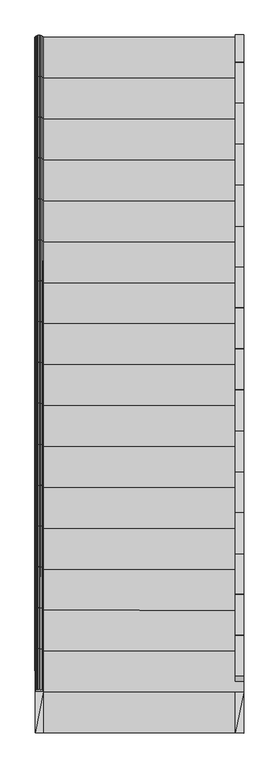
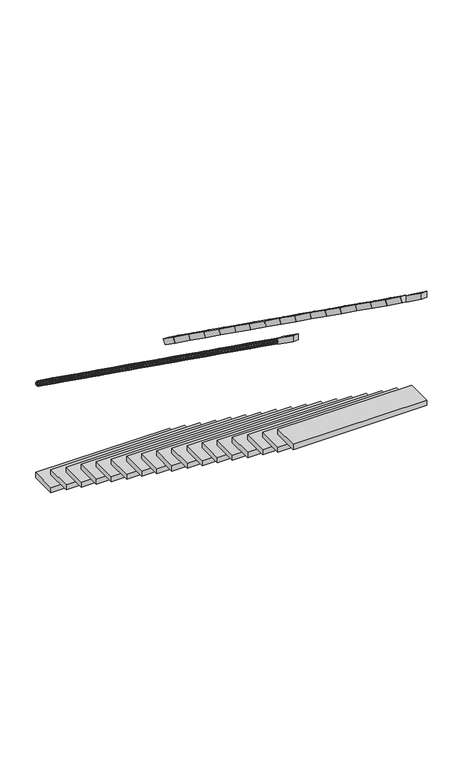
"""IFC4 building model written with IfcOpenShell, lengths in millimetres: stair geometry, 0_3d_modell."""

from ifc_helpers import new_model, si_unit, frame, origin, origin_with_axes, place, context, project, spatial, polyline, outline, extrude, faceted_brep, source, transform, mapped, element, save


def stair_c8e6e2fb(model_context):
    return source(origin(), model_context, "Body", "SolidModel", [
        extrude(outline(polyline([(1249.8201376, 2937.4233037), (1249.7841678, 2692.4712959), (0.2158186, 2693.7650028), (0.1798488, 2938.4708402), (1249.8201376, 2937.4233037)])), frame((0.0, 0.0, 875.0), z_axis=(0.0, 0.0, 1.0), x_axis=(1.0, 0.0, 0.0)), (0.0, 0.0, 1.0), 50.0),
        faceted_brep([(1.6558478, 1221.2875213, 3015.1503975), (0.4316459, 1225.4705658, 3021.0), (1.654618, 1229.65397, 3026.8496025), (5.2050513, 1233.4282332, 3032.1266051), (10.7354046, 1236.4239042, 3036.3144581), (17.7043284, 1238.3477458, 3039.0032253), (25.4296557, 1239.011439, 3039.9297113), (33.1551779, 1238.3500169, 3039.0032253), (40.1246669, 1236.4282241, 3036.3144581), (45.6559006, 1233.4341791, 3032.1266051), (49.2074433, 1229.6609599, 3026.8496025), (50.4316453, 1225.4779154, 3021.0), (49.2086731, 1221.2945111, 3015.1503975), (45.6582398, 1217.520248, 3009.8733949), (40.1278866, 1214.524577, 3005.6855419), (33.1589628, 1212.6007354, 3002.9967747), (25.4336355, 1211.9370421, 3002.0702887), (17.7081133, 1212.5984642, 3002.9967747), (10.7386243, 1214.520257, 3005.6855419), (5.2073906, 1217.514302, 3009.8733949), (1.6905885, 984.9431074, 3201.8496026), (0.4676164, 980.7597033, 3196.0), (1.6918183, 976.5766589, 3190.1503974), (5.2433611, 972.8034398, 3184.8733946), (10.7745948, 969.8093949, 3180.6855416), (17.7440838, 967.8876022, 3177.9967744), (25.469606, 967.2261802, 3177.0702883), (33.1949333, 967.8898734, 3177.9967744), (40.1638571, 969.8137149, 3180.6855416), (45.6942103, 972.8093858, 3184.8733946), (49.2446436, 976.5836488, 3190.1503974), (50.4676158, 980.7670529, 3196.0), (49.2434138, 984.9500972, 3201.8496026), (45.6918711, 988.7233163, 3207.1266054), (40.1606374, 991.7173612, 3211.3144584), (33.1911484, 993.6391539, 3214.0032256), (25.4656262, 994.300576, 3214.9297117), (17.7402989, 993.6368828, 3214.0032256), (10.7713751, 991.7130413, 3211.3144584), (5.2410218, 988.7173704, 3207.1266054)], [[[0, 1, 2, 3, 4, 5, 6, 7, 8, 9, 10, 11, 12, 13, 14, 15, 16, 17, 18, 19]], [[20, 21, 22, 23, 24, 25, 26, 27, 28, 29, 30, 31, 32, 33, 34, 35, 36, 37, 38, 39]], [[2, 1, 21, 20]], [[3, 2, 20, 39]], [[4, 3, 39, 38]], [[5, 4, 38, 37]], [[6, 5, 37, 36]], [[7, 6, 36, 35]], [[8, 7, 35, 34]], [[9, 8, 34, 33]], [[10, 9, 33, 32]], [[11, 10, 32, 31]], [[12, 11, 31, 30]], [[13, 12, 30, 29]], [[14, 13, 29, 28]], [[15, 14, 28, 27]], [[16, 15, 27, 26]], [[17, 16, 26, 25]], [[18, 17, 25, 24]], [[19, 18, 24, 23]], [[0, 19, 23, 22]], [[1, 0, 22, 21]]]),
        extrude(outline(polyline([(8.1923594, -49.3242866), (0.0, 0.0), (296.970001, 49.3242865), (305.1623617, 2e-07), (8.1923594, -49.3242866)])), frame((1249.7982535, 2788.3939483, 1932.2457474), z_axis=(-0.9999999892183942, 0.00014684417532646174, 0.0), x_axis=(-0.00013185516429988818, -0.8979257278461469, 0.44014698668306607)), (0.0, 0.0, 1.0), 50.0),
        extrude(outline(polyline([(8.1923603, -49.3242865), (0.0, 0.0), (296.9699661, 49.3242863), (305.1623277, 1e-07), (8.1923603, -49.3242865)])), frame((1249.6903463, 2053.5527853, 2457.2457396), z_axis=(-0.9999999892183942, 0.00014684417532705656, 0.0), x_axis=(-0.00013185516035039472, -0.897925700001221, 0.44014704348834854)), (0.0, 0.0, 1.0), 50.0),
        faceted_brep([(1.7637594, 487.1548921, 3540.1503972), (0.5395574, 491.3379361, 3546.0), (1.7625296, 495.5213399, 3551.8496028), (5.3129629, 499.2956026, 3557.1266058), (10.8433161, 502.2912733, 3561.314459), (17.8122399, 504.2151146, 3564.0032263), (25.5375672, 504.8788078, 3564.9297124), (33.2630894, 504.2173858, 3564.0032263), (40.2325784, 502.2955932, 3561.314459), (45.7638121, 499.3015486, 3557.1266058), (49.3153549, 495.5283297, 3551.8496028), (50.5395568, 491.3452857, 3546.0), (49.3165847, 487.161882, 3540.1503972), (45.7661514, 483.3876192, 3534.8733942), (40.2357981, 480.3919486, 3530.685541), (33.2668743, 478.4681072, 3527.9967737), (25.541547, 477.804414, 3527.0702876), (17.8160248, 478.465836, 3527.9967737), (10.8465358, 480.3876286, 3530.685541), (5.3153021, 483.3816732, 3534.8733942), (1.7985001, 250.810435, 3726.8496029), (0.5755279, 246.6270315, 3721.0), (1.7997299, 242.4439876, 3715.1503971), (5.3512726, 238.6707689, 3709.873394), (10.8825063, 235.6767243, 3705.6855407), (17.8519953, 233.7549319, 3702.9967733), (25.5775175, 233.0935099, 3702.0702872), (33.3028449, 233.757203, 3702.9967733), (40.2717686, 235.6810443, 3705.6855407), (45.8021219, 238.6767148, 3709.873394), (49.3525552, 242.4509775, 3715.1503971), (50.5755273, 246.634381, 3721.0), (49.3513254, 250.8174249, 3726.8496029), (45.7997826, 254.5906436, 3732.126606), (40.2685489, 257.5846882, 3736.3144593), (33.2990599, 259.5064806, 3739.0032267), (25.5735378, 260.1679026, 3739.9297128), (17.8482104, 259.5042095, 3739.0032267), (10.8792866, 257.5803682, 3736.3144593), (5.3489334, 254.5846977, 3732.126606)], [[[0, 1, 2, 3, 4, 5, 6, 7, 8, 9, 10, 11, 12, 13, 14, 15, 16, 17, 18, 19]], [[20, 21, 22, 23, 24, 25, 26, 27, 28, 29, 30, 31, 32, 33, 34, 35, 36, 37, 38, 39]], [[2, 1, 21, 20]], [[3, 2, 20, 39]], [[4, 3, 39, 38]], [[5, 4, 38, 37]], [[6, 5, 37, 36]], [[7, 6, 36, 35]], [[8, 7, 35, 34]], [[9, 8, 34, 33]], [[10, 9, 33, 32]], [[11, 10, 32, 31]], [[12, 11, 31, 30]], [[13, 12, 30, 29]], [[14, 13, 29, 28]], [[15, 14, 28, 27]], [[16, 15, 27, 26]], [[17, 16, 26, 25]], [[18, 17, 25, 24]], [[19, 18, 24, 23]], [[0, 19, 23, 22]], [[1, 0, 22, 21]]]),
        extrude(outline(polyline([(8.1923606, -49.3242864), (0.0, 0.0), (296.9699544, 49.3242862), (305.1623164, 1e-07), (8.1923606, -49.3242864)])), frame((1249.6543773, 1808.6057592, 2632.245737), z_axis=(-0.9999999892183942, 0.00014684417504094816, 0.0), x_axis=(-0.0001318551587321288, -0.8979256907316214, 0.4401470623988734)), (0.0, 0.0, 1.0), 50.0),
        faceted_brep([(1.3321134, 3423.6846479, 1440.1503985), (0.1079114, 3427.8676939, 1446.0), (1.3308836, 3432.0510995, 1451.8496015), (4.8813169, 3435.825364, 1457.1266032), (10.4116702, 3438.821036, 1461.3144555), (17.3805939, 3440.7448783, 1464.0032221), (25.1059213, 3441.4085717, 1464.929708), (32.8314435, 3440.7471494, 1464.0032221), (39.8009325, 3438.825356, 1461.3144555), (45.3321662, 3435.8313099, 1457.1266032), (48.8837089, 3432.0580894, 1451.8496015), (50.1079109, 3427.8750434, 1446.0), (48.8849387, 3423.6916378, 1440.1503985), (45.3345054, 3419.9173733, 1434.8733968), (39.8041521, 3416.9217013, 1430.6855445), (32.8352284, 3414.997859, 1427.9967779), (25.109901, 3414.3341656, 1427.070292), (17.3843789, 3414.9955879, 1427.9967779), (10.4148898, 3416.9173813, 1430.6855445), (4.8836561, 3419.9114273, 1434.8733968), (1.3668541, 3187.3403638, 1626.8496016), (0.1438819, 3183.1569583, 1621.0), (1.3680839, 3178.9739126, 1615.1503984), (4.9196266, 3175.2006921, 1609.8733966), (10.4508603, 3172.2066462, 1605.6855442), (17.4203493, 3170.2848529, 1602.9967775), (25.1458715, 3169.6234306, 1602.0702916), (32.8711989, 3170.287124, 1602.9967775), (39.8401226, 3172.2109662, 1605.6855442), (45.3704759, 3175.2066381, 1609.8733966), (48.9209092, 3178.9809024, 1615.1503984), (50.1438814, 3183.1643079, 1621.0), (48.9196794, 3187.3473537, 1626.8496016), (45.3681367, 3191.1205741, 1632.1266034), (39.836903, 3194.1146201, 1636.3144558), (32.867414, 3196.0364134, 1639.0032225), (25.1418918, 3196.6978357, 1639.9297084), (17.4165644, 3196.0341423, 1639.0032225), (10.4476407, 3194.1103001, 1636.3144558), (4.9172874, 3191.1146282, 1632.1266034)], [[[0, 1, 2, 3, 4, 5, 6, 7, 8, 9, 10, 11, 12, 13, 14, 15, 16, 17, 18, 19]], [[20, 21, 22, 23, 24, 25, 26, 27, 28, 29, 30, 31, 32, 33, 34, 35, 36, 37, 38, 39]], [[2, 1, 21, 20]], [[3, 2, 20, 39]], [[4, 3, 39, 38]], [[5, 4, 38, 37]], [[6, 5, 37, 36]], [[7, 6, 36, 35]], [[8, 7, 35, 34]], [[9, 8, 34, 33]], [[10, 9, 33, 32]], [[11, 10, 32, 31]], [[12, 11, 31, 30]], [[13, 12, 30, 29]], [[14, 13, 29, 28]], [[15, 14, 28, 27]], [[16, 15, 27, 26]], [[17, 16, 26, 25]], [[18, 17, 25, 24]], [[19, 18, 24, 23]], [[0, 19, 23, 22]], [[1, 0, 22, 21]]]),
        faceted_brep([(0.6114861, 0.0837476, 3867.0), (0.5755163, 246.7058527, 3692.0), (50.5755389, 246.5555598, 3692.0), (50.6115102, 0.0, 3867.0), (50.5755389, 246.5555598, 3750.0), (0.5755163, 246.7058527, 3750.0), (0.6114861, 0.0837476, 3925.0), (50.6115102, 0.0, 3925.0)], [[[0, 1, 2]], [[3, 0, 2]], [[4, 5, 6]], [[7, 4, 6]], [[4, 2, 1, 5]], [[5, 1, 0, 6]], [[6, 0, 3, 7]], [[7, 3, 2, 4]]]),
        faceted_brep([(1.2961429, 3668.3953691, 1265.1503986), (0.071941, 3672.5784152, 1271.0), (1.2949131, 3676.761821, 1276.8496014), (4.8453464, 3680.5360857, 1282.126603), (10.3756997, 3683.5317578, 1286.3144552), (17.3446234, 3685.4556001, 1289.0032218), (25.0699508, 3686.1192936, 1289.9297076), (32.795473, 3685.4578713, 1289.0032218), (39.764962, 3683.5360778, 1286.3144552), (45.2961957, 3680.5420316, 1282.126603), (48.8477384, 3676.7688109, 1276.8496014), (50.0719404, 3672.5857648, 1271.0), (48.8489682, 3668.402359, 1265.1503986), (45.2985349, 3664.6280943, 1259.873397), (39.7681817, 3661.6324222, 1255.6855448), (32.7992579, 3659.7085799, 1252.9967782), (25.0739305, 3659.0448864, 1252.0702924), (17.3484084, 3659.7063087, 1252.9967782), (10.3789194, 3661.6281022, 1255.6855448), (4.8476857, 3664.6221484, 1259.873397), (1.3308836, 3432.0510995, 1451.8496015), (0.1079114, 3427.8676939, 1446.0), (1.3321134, 3423.6846479, 1440.1503985), (4.8836561, 3419.9114273, 1434.8733968), (10.4148898, 3416.9173813, 1430.6855445), (17.3843789, 3414.9955879, 1427.9967779), (25.109901, 3414.3341656, 1427.070292), (32.8352284, 3414.997859, 1427.9967779), (39.8041521, 3416.9217013, 1430.6855445), (45.3345054, 3419.9173733, 1434.8733968), (48.8849387, 3423.6916378, 1440.1503985), (50.1079109, 3427.8750434, 1446.0), (48.8837089, 3432.0580894, 1451.8496015), (45.3321662, 3435.8313099, 1457.1266032), (39.8009325, 3438.825356, 1461.3144555), (32.8314435, 3440.7471494, 1464.0032221), (25.1059213, 3441.4085717, 1464.929708), (17.3805939, 3440.7448783, 1464.0032221), (10.4116702, 3438.821036, 1461.3144555), (4.8813169, 3435.825364, 1457.1266032)], [[[0, 1, 2, 3, 4, 5, 6, 7, 8, 9, 10, 11, 12, 13, 14, 15, 16, 17, 18, 19]], [[20, 21, 22, 23, 24, 25, 26, 27, 28, 29, 30, 31, 32, 33, 34, 35, 36, 37, 38, 39]], [[2, 1, 21, 20]], [[3, 2, 20, 39]], [[4, 3, 39, 38]], [[5, 4, 38, 37]], [[6, 5, 37, 36]], [[7, 6, 36, 35]], [[8, 7, 35, 34]], [[9, 8, 34, 33]], [[10, 9, 33, 32]], [[11, 10, 32, 31]], [[12, 11, 31, 30]], [[13, 12, 30, 29]], [[14, 13, 29, 28]], [[15, 14, 28, 27]], [[16, 15, 27, 26]], [[17, 16, 26, 25]], [[18, 17, 25, 24]], [[19, 18, 24, 23]], [[0, 19, 23, 22]], [[1, 0, 22, 21]]]),
        extrude(outline(polyline([(8.1923617, -49.3242862), (0.0, 0.0), (296.9699081, 49.3242861), (305.1622712, 1e-07), (8.1923617, -49.3242862)])), frame((1249.5105011, 828.8177955, 3332.2457265), z_axis=(-0.9999999892183942, 0.00014684417525931187, 0.0), x_axis=(-0.00013185515344095938, -0.8979256537134775, 0.4401471379180406)), (0.0, 0.0, 1.0), 50.0),
        extrude(outline(polyline([(8.1923621, -49.3242861), (0.0, 0.0), (296.9698965, 49.324286), (305.16226, 1e-07), (8.1923621, -49.3242861)])), frame((1249.4745321, 583.8708398, 3507.2457239), z_axis=(-0.9999999892183941, 0.0001468441754534332, 0.0), x_axis=(-0.00013185515234816458, -0.8979256444740151, 0.4401471567670788)), (0.0, 0.0, 1.0), 50.0),
        extrude(outline(polyline([(8.1923599, -49.3242865), (0.0, 0.0), (296.9699777, 49.3242864), (305.162339, 1e-07), (8.1923599, -49.3242865)])), frame((1249.7263154, 2298.4998255, 2282.2457422), z_axis=(-0.9999999892183941, 0.00014684417517801771, 0.0), x_axis=(-0.00013185516162205705, -0.8979257092768325, 0.44014702456555777)), (0.0, 0.0, 1.0), 50.0),
        extrude(outline(polyline([(1249.4604399, 487.9038597), (1249.4244702, 242.9519926), (0.5755163, 246.7058527), (0.5395465, 491.411831), (1249.4604399, 487.9038597)])), frame((0.0, 0.0, 2625.0), z_axis=(0.0, 0.0, 1.0), x_axis=(1.0, 0.0, 0.0)), (0.0, 0.0, 1.0), 50.0),
        extrude(outline(polyline([(8.1923597, -49.3242865), (0.0, 0.0), (296.9699893, 49.3242865), (305.1623503, 1e-07), (8.1923597, -49.3242865)])), frame((1249.7622844, 2543.4468798, 2107.2457448), z_axis=(-0.9999999892183941, 0.00014684417524442892, 0.0), x_axis=(-0.00013185516302004327, -0.8979257185584691, 0.4401470056304744)), (0.0, 0.0, 1.0), 50.0),
        extrude(outline(polyline([(1249.8920771, 3427.3273618), (1249.8561074, 3182.3753257), (0.143879, 3183.1766636), (0.1079093, 3427.8824728), (1249.8920771, 3427.3273618)])), frame((0.0, 0.0, 525.0), z_axis=(0.0, 0.0, 1.0), x_axis=(1.0, 0.0, 0.0)), (0.0, 0.0, 1.0), 50.0),
        extrude(outline(polyline([(1249.4244702, 242.9519926), (1249.3885004, 0.0), (0.6114861, 0.0837476), (0.5755163, 246.7058527), (1249.4244702, 242.9519926)])), frame((0.0, 0.0, 2800.0), z_axis=(0.0, 0.0, 1.0), x_axis=(1.0, 0.0, 0.0)), (0.0, 0.0, 1.0), 50.0),
        extrude(outline(polyline([(1249.7841678, 2692.4712959), (1249.748198, 2447.5193021), (0.2517883, 2449.0591512), (0.2158186, 2693.7650028), (1249.7841678, 2692.4712959)])), frame((0.0, 0.0, 1050.0), z_axis=(0.0, 0.0, 1.0), x_axis=(1.0, 0.0, 0.0)), (0.0, 0.0, 1.0), 50.0),
        extrude(outline(polyline([(1249.604319, 1467.7114683), (1249.5683492, 1222.759545), (0.4316372, 1225.5296816), (0.3956674, 1470.2356037), (1249.604319, 1467.7114683)])), frame((0.0, 0.0, 1925.0), z_axis=(0.0, 0.0, 1.0), x_axis=(1.0, 0.0, 0.0)), (0.0, 0.0, 1.0), 50.0),
        extrude(outline(polyline([(1249.6402887, 1712.6634056), (1249.604319, 1467.7114683), (0.3956674, 1470.2356037), (0.3596976, 1714.9415117), (1249.6402887, 1712.6634056)])), frame((0.0, 0.0, 1750.0), z_axis=(0.0, 0.0, 1.0), x_axis=(1.0, 0.0, 0.0)), (0.0, 0.0, 1.0), 50.0),
        extrude(outline(polyline([(1249.8561074, 3182.3753257), (1249.8201376, 2937.4233037), (0.1798488, 2938.4708402), (0.143879, 3183.1766636), (1249.8561074, 3182.3753257)])), frame((0.0, 0.0, 700.0), z_axis=(0.0, 0.0, 1.0), x_axis=(1.0, 0.0, 0.0)), (0.0, 0.0, 1.0), 50.0),
        faceted_brep([(1.4759954, 2444.8416217, 2140.1503981), (0.2517934, 2449.024667, 2146.0), (1.4747656, 2453.208072, 2151.8496019), (5.0251989, 2456.9823359, 2157.1266041), (10.5555521, 2459.9780075, 2161.3144567), (17.5244759, 2461.9018494, 2164.0032235), (25.2498033, 2462.5655428, 2164.9297095), (32.9753254, 2461.9041206, 2164.0032235), (39.9448144, 2459.9823274, 2161.3144567), (45.4760481, 2456.9882819, 2157.1266041), (49.0275909, 2453.2150619, 2151.8496019), (50.2517928, 2449.0320166, 2146.0), (49.0288207, 2444.8486115, 2140.1503981), (45.4783874, 2441.0743476, 2134.8733959), (39.9480341, 2438.0786761, 2130.6855433), (32.9791104, 2436.1548341, 2127.9967765), (25.253783, 2435.4911408, 2127.0702905), (17.5282608, 2436.152563, 2127.9967765), (10.5587718, 2438.0743561, 2130.6855433), (5.0275381, 2441.0684017, 2134.8733959), (1.5107361, 2208.4972798, 2326.849602), (0.2877639, 2204.3138749, 2321.0), (1.5119659, 2200.1308298, 2315.150398), (5.0635086, 2196.35761, 2309.8733957), (10.5947423, 2193.3635645, 2305.685543), (17.5642313, 2191.4417714, 2302.9967761), (25.2897535, 2190.7803492, 2302.0702902), (33.0150808, 2191.4440426, 2302.9967761), (39.9840046, 2193.3678845, 2305.685543), (45.5143579, 2196.3635559, 2309.8733957), (49.0647912, 2200.1378197, 2315.150398), (50.2877633, 2204.3212245, 2321.0), (49.0635614, 2208.5042697, 2326.849602), (45.5120186, 2212.2774895, 2332.1266043), (39.9807849, 2215.271535, 2336.314457), (33.0112959, 2217.193328, 2339.0032239), (25.2857737, 2217.8547502, 2339.9297098), (17.5604464, 2217.1910569, 2339.0032239), (10.5915226, 2215.267215, 2336.314457), (5.0611694, 2212.2715436, 2332.1266043)], [[[0, 1, 2, 3, 4, 5, 6, 7, 8, 9, 10, 11, 12, 13, 14, 15, 16, 17, 18, 19]], [[20, 21, 22, 23, 24, 25, 26, 27, 28, 29, 30, 31, 32, 33, 34, 35, 36, 37, 38, 39]], [[2, 1, 21, 20]], [[3, 2, 20, 39]], [[4, 3, 39, 38]], [[5, 4, 38, 37]], [[6, 5, 37, 36]], [[7, 6, 36, 35]], [[8, 7, 35, 34]], [[9, 8, 34, 33]], [[10, 9, 33, 32]], [[11, 10, 32, 31]], [[12, 11, 31, 30]], [[13, 12, 30, 29]], [[14, 13, 29, 28]], [[15, 14, 28, 27]], [[16, 15, 27, 26]], [[17, 16, 26, 25]], [[18, 17, 25, 24]], [[19, 18, 24, 23]], [[0, 19, 23, 22]], [[1, 0, 22, 21]]]),
        extrude(outline(polyline([(8.1923588, -49.3242867), (0.0, 0.0), (296.9700243, 49.3242866), (305.1623845, 1e-07), (8.1923588, -49.3242867)])), frame((1249.8701916, 3278.2881276, 1582.2457526), z_axis=(-0.9999999892183941, 0.0001468441752435612, 0.0), x_axis=(-0.0001318551671803848, -0.8979257464395893, 0.44014694875134736)), (0.0, 0.0, 1.0), 50.0),
        extrude(outline(polyline([(1249.9640167, 3917.2314766), (1249.9280469, 3672.2794121), (0.0719395, 3672.5882678), (0.0359698, 3917.2940487), (1249.9640167, 3917.2314766)])), frame((0.0, 0.0, 175.0), z_axis=(0.0, 0.0, 1.0), x_axis=(1.0, 0.0, 0.0)), (0.0, 0.0, 1.0), 50.0),
        faceted_brep([(1.3680839, 3178.9739126, 1615.1503984), (0.1438819, 3183.1569583, 1621.0), (1.3668541, 3187.3403638, 1626.8496016), (4.9172874, 3191.1146282, 1632.1266034), (10.4476407, 3194.1103001, 1636.3144558), (17.4165644, 3196.0341423, 1639.0032225), (25.1418918, 3196.6978357, 1639.9297084), (32.867414, 3196.0364134, 1639.0032225), (39.836903, 3194.1146201, 1636.3144558), (45.3681367, 3191.1205741, 1632.1266034), (48.9196794, 3187.3473537, 1626.8496016), (50.1438814, 3183.1643079, 1621.0), (48.9209092, 3178.9809024, 1615.1503984), (45.3704759, 3175.2066381, 1609.8733966), (39.8401226, 3172.2109662, 1605.6855442), (32.8711989, 3170.287124, 1602.9967775), (25.1458715, 3169.6234306, 1602.0702916), (17.4203493, 3170.2848529, 1602.9967775), (10.4508603, 3172.2066462, 1605.6855442), (4.9196266, 3175.2006921, 1609.8733966), (1.4028246, 2942.629614, 1801.8496017), (0.1798524, 2938.4462087, 1796.0), (1.4040544, 2934.2631631, 1790.1503983), (4.9555971, 2930.4899428, 1784.8733964), (10.4868308, 2927.495897, 1780.6855439), (17.4563198, 2925.5741037, 1777.9967772), (25.181842, 2924.9126814, 1777.0702913), (32.9071694, 2925.5763748, 1777.9967772), (39.8760931, 2927.500217, 1780.6855439), (45.4064464, 2930.4958887, 1784.8733964), (48.9568797, 2934.2701529, 1790.1503983), (50.1798519, 2938.4535583, 1796.0), (48.9556499, 2942.6366039, 1801.8496017), (45.4041072, 2946.4098242, 1807.1266036), (39.8728735, 2949.40387, 1811.3144561), (32.9033844, 2951.3256633, 1814.0032228), (25.1778623, 2951.9870855, 1814.9297087), (17.4525349, 2951.3233921, 1814.0032228), (10.4836112, 2949.39955, 1811.3144561), (4.9532579, 2946.4038782, 1807.1266036)], [[[0, 1, 2, 3, 4, 5, 6, 7, 8, 9, 10, 11, 12, 13, 14, 15, 16, 17, 18, 19]], [[20, 21, 22, 23, 24, 25, 26, 27, 28, 29, 30, 31, 32, 33, 34, 35, 36, 37, 38, 39]], [[2, 1, 21, 20]], [[3, 2, 20, 39]], [[4, 3, 39, 38]], [[5, 4, 38, 37]], [[6, 5, 37, 36]], [[7, 6, 36, 35]], [[8, 7, 35, 34]], [[9, 8, 34, 33]], [[10, 9, 33, 32]], [[11, 10, 32, 31]], [[12, 11, 31, 30]], [[13, 12, 30, 29]], [[14, 13, 29, 28]], [[15, 14, 28, 27]], [[16, 15, 27, 26]], [[17, 16, 26, 25]], [[18, 17, 25, 24]], [[19, 18, 24, 23]], [[0, 19, 23, 22]], [[1, 0, 22, 21]]]),
        faceted_brep([(1.4040544, 2934.2631631, 1790.1503983), (0.1798524, 2938.4462087, 1796.0), (1.4028246, 2942.629614, 1801.8496017), (4.9532579, 2946.4038782, 1807.1266036), (10.4836112, 2949.39955, 1811.3144561), (17.4525349, 2951.3233921, 1814.0032228), (25.1778623, 2951.9870855, 1814.9297087), (32.9033844, 2951.3256633, 1814.0032228), (39.8728735, 2949.40387, 1811.3144561), (45.4041072, 2946.4098242, 1807.1266036), (48.9556499, 2942.6366039, 1801.8496017), (50.1798519, 2938.4535583, 1796.0), (48.9568797, 2934.2701529, 1790.1503983), (45.4064464, 2930.4958887, 1784.8733964), (39.8760931, 2927.500217, 1780.6855439), (32.9071694, 2925.5763748, 1777.9967772), (25.181842, 2924.9126814, 1777.0702913), (17.4563198, 2925.5741037, 1777.9967772), (10.4868308, 2927.495897, 1780.6855439), (4.9555971, 2930.4899428, 1784.8733964), (1.4387951, 2697.9188501, 1976.8496018), (0.2158229, 2693.7354449, 1971.0), (1.4400249, 2689.5523994, 1965.1503982), (4.9915676, 2685.7791793, 1959.8733962), (10.5228013, 2682.7851336, 1955.6855436), (17.4922903, 2680.8633404, 1952.9967768), (25.2178125, 2680.2019182, 1952.0702909), (32.9431399, 2680.8656115, 1952.9967768), (39.9120636, 2682.7894536, 1955.6855436), (45.4424169, 2685.7851253, 1959.8733962), (48.9928502, 2689.5593893, 1965.1503982), (50.2158224, 2693.7427945, 1971.0), (48.9916204, 2697.92584, 1976.8496018), (45.4400777, 2701.6990601, 1982.1266038), (39.9088439, 2704.6931058, 1986.3144564), (32.9393549, 2706.614899, 1989.0032232), (25.2138328, 2707.2763212, 1989.9297091), (17.4885054, 2706.6126278, 1989.0032232), (10.5195816, 2704.6887858, 1986.3144564), (4.9892284, 2701.6931141, 1982.1266038)], [[[0, 1, 2, 3, 4, 5, 6, 7, 8, 9, 10, 11, 12, 13, 14, 15, 16, 17, 18, 19]], [[20, 21, 22, 23, 24, 25, 26, 27, 28, 29, 30, 31, 32, 33, 34, 35, 36, 37, 38, 39]], [[2, 1, 21, 20]], [[3, 2, 20, 39]], [[4, 3, 39, 38]], [[5, 4, 38, 37]], [[6, 5, 37, 36]], [[7, 6, 36, 35]], [[8, 7, 35, 34]], [[9, 8, 34, 33]], [[10, 9, 33, 32]], [[11, 10, 32, 31]], [[12, 11, 31, 30]], [[13, 12, 30, 29]], [[14, 13, 29, 28]], [[15, 14, 28, 27]], [[16, 15, 27, 26]], [[17, 16, 26, 25]], [[18, 17, 25, 24]], [[19, 18, 24, 23]], [[0, 19, 23, 22]], [[1, 0, 22, 21]]]),
        extrude(outline(polyline([(8.1923612, -49.3242862), (0.0, 0.0), (296.9699313, 49.3242862), (305.1622938, 1e-07), (8.1923612, -49.3242862)])), frame((1249.5824392, 1318.7117492, 2982.2457317), z_axis=(-0.9999999892183942, 0.0001468441753559752, 0.0), x_axis=(-0.00013185515634028903, -0.8979256722105143, 0.4401471001830111)), (0.0, 0.0, 1.0), 50.0),
        faceted_brep([(1.5479363, 1955.4200238, 2490.1503978), (0.3237344, 1959.6030688, 2496.0), (1.5467065, 1963.7864735, 2501.8496022), (5.0971398, 1967.5607371, 2507.1266045), (10.6274931, 1970.5564084, 2511.3144573), (17.5964169, 1972.4802503, 2514.0032242), (25.3217442, 1973.1439436, 2514.9297102), (33.0472664, 1972.4825214, 2514.0032242), (40.0167554, 1970.5607284, 2511.3144573), (45.5479891, 1967.5666831, 2507.1266045), (49.0995319, 1963.7934634, 2501.8496022), (50.3237338, 1959.6104184, 2496.0), (49.1007617, 1955.4270137, 2490.1503978), (45.5503284, 1951.6527501, 2484.8733955), (40.0199751, 1948.6570787, 2480.6855427), (33.0510513, 1946.7332369, 2477.9967758), (25.325724, 1946.0695436, 2477.0702898), (17.6002018, 1946.7309658, 2477.9967758), (10.6307128, 1948.6527588, 2480.6855427), (5.0994791, 1951.6468041, 2484.8733955), (1.582677, 1719.0756531, 2676.8496023), (0.3597049, 1714.8922485, 2671.0), (1.5839068, 1710.7092037, 2665.1503977), (5.1354496, 1706.9359842, 2659.8733953), (10.6666833, 1703.9419389, 2655.6855424), (17.6361723, 1702.020146, 2652.9967754), (25.3616945, 1701.3587239, 2652.0702894), (33.0870218, 1702.0224172, 2652.9967754), (40.0559456, 1703.9462589, 2655.6855424), (45.5862988, 1706.9419301, 2659.8733953), (49.1367321, 1710.7161936, 2665.1503977), (50.3597043, 1714.8995981, 2671.0), (49.1355023, 1719.082643, 2676.8496023), (45.5839596, 1722.8558625, 2682.1266047), (40.0527259, 1725.8499077, 2686.3144576), (33.0832369, 1727.7717007, 2689.0032246), (25.3577147, 1728.4331228, 2689.9297106), (17.6323874, 1727.7694295, 2689.0032246), (10.6634636, 1725.8455878, 2686.3144576), (5.1331103, 1722.8499166, 2682.1266047)], [[[0, 1, 2, 3, 4, 5, 6, 7, 8, 9, 10, 11, 12, 13, 14, 15, 16, 17, 18, 19]], [[20, 21, 22, 23, 24, 25, 26, 27, 28, 29, 30, 31, 32, 33, 34, 35, 36, 37, 38, 39]], [[2, 1, 21, 20]], [[3, 2, 20, 39]], [[4, 3, 39, 38]], [[5, 4, 38, 37]], [[6, 5, 37, 36]], [[7, 6, 36, 35]], [[8, 7, 35, 34]], [[9, 8, 34, 33]], [[10, 9, 33, 32]], [[11, 10, 32, 31]], [[12, 11, 31, 30]], [[13, 12, 30, 29]], [[14, 13, 29, 28]], [[15, 14, 28, 27]], [[16, 15, 27, 26]], [[17, 16, 26, 25]], [[18, 17, 25, 24]], [[19, 18, 24, 23]], [[0, 19, 23, 22]], [[1, 0, 22, 21]]]),
        extrude(outline(polyline([(1249.5683492, 1222.759545), (1249.5323794, 977.8076359), (0.467607, 980.8237455), (0.4316372, 1225.5296816), (1249.5683492, 1222.759545)])), frame((0.0, 0.0, 2100.0), z_axis=(0.0, 0.0, 1.0), x_axis=(1.0, 0.0, 0.0)), (0.0, 0.0, 1.0), 50.0),
        extrude(outline(polyline([(8.1923585, -49.3242867), (0.0, 0.0), (296.9700358, 49.3242866), (305.1623956, 1e-07), (8.1923585, -49.3242867)])), frame((1249.9061607, 3523.2352384, 1407.2457553), z_axis=(-0.9999999892183941, 0.0001468441750096529, 0.0), x_axis=(-0.00013185516823967282, -0.8979257557453386, 0.44014692976706893)), (0.0, 0.0, 1.0), 50.0),
        extrude(outline(polyline([(1249.4964097, 732.8557407), (1249.4604399, 487.9038597), (0.5395465, 491.411831), (0.5035767, 736.1177952), (1249.4964097, 732.8557407)])), frame((0.0, 0.0, 2450.0), z_axis=(0.0, 0.0, 1.0), x_axis=(1.0, 0.0, 0.0)), (0.0, 0.0, 1.0), 50.0),
        extrude(outline(polyline([(8.1923581, -49.3242868), (0.0, 0.0), (296.9700476, 49.3242867), (305.1624071, 1e-07), (8.1923581, -49.3242868)])), frame((1249.9421297, 3768.1823634, 1232.2457579), z_axis=(-0.9999999892183941, 0.0001468441755103031, 0.0), x_axis=(-0.0001318551699986651, -0.8979257650571624, 0.44014691077039697)), (0.0, 0.0, 1.0), 50.0),
        extrude(outline(polyline([(8.1923579, -49.3242869), (0.0, 0.0), (296.9700593, 49.3242867), (305.1624184, 2e-07), (8.1923579, -49.3242869)])), frame((1249.9780988, 4013.1295026, 1057.2457605), z_axis=(-0.9999999892183941, 0.00014684417562510396, 0.0), x_axis=(-0.00013185517137757034, -0.8979257743750024, 0.4401468917614504)), (0.0, 0.0, 1.0), 50.0),
        faceted_brep([(1.6918183, 976.5766589, 3190.1503974), (0.4676164, 980.7597033, 3196.0), (1.6905885, 984.9431074, 3201.8496026), (5.2410218, 988.7173704, 3207.1266054), (10.7713751, 991.7130413, 3211.3144584), (17.7402989, 993.6368828, 3214.0032256), (25.4656262, 994.300576, 3214.9297117), (33.1911484, 993.6391539, 3214.0032256), (40.1606374, 991.7173612, 3211.3144584), (45.6918711, 988.7233163, 3207.1266054), (49.2434138, 984.9500972, 3201.8496026), (50.4676158, 980.7670529, 3196.0), (49.2446436, 976.5836488, 3190.1503974), (45.6942103, 972.8093858, 3184.8733946), (40.1638571, 969.8137149, 3180.6855416), (33.1949333, 967.8898734, 3177.9967744), (25.469606, 967.2261802, 3177.0702883), (17.7440838, 967.8876022, 3177.9967744), (10.7745948, 969.8093949, 3180.6855416), (5.2433611, 972.8034398, 3184.8733946), (1.7265591, 740.2322306, 3376.8496027), (0.5035869, 736.0488267, 3371.0), (1.7277888, 731.8657825, 3365.1503973), (5.2793316, 728.0925636, 3359.8733944), (10.8105653, 725.0985188, 3355.6855413), (17.7800543, 723.1767261, 3352.996774), (25.5055765, 722.5153041, 3352.070288), (33.2309038, 723.1789973, 3352.996774), (40.1998276, 725.1028388, 3355.6855413), (45.7301809, 728.0985095, 3359.8733944), (49.2806142, 731.8727724, 3365.1503973), (50.5035863, 736.0561763, 3371.0), (49.2793844, 740.2392205, 3376.8496027), (45.7278416, 744.0124395, 3382.1266056), (40.1966079, 747.0064843, 3386.3144587), (33.2271189, 748.9282769, 3389.003226), (25.5015967, 749.5896989, 3389.929712), (17.7762694, 748.9260057, 3389.003226), (10.8073456, 747.0021643, 3386.3144587), (5.2769924, 744.0064935, 3382.1266056)], [[[0, 1, 2, 3, 4, 5, 6, 7, 8, 9, 10, 11, 12, 13, 14, 15, 16, 17, 18, 19]], [[20, 21, 22, 23, 24, 25, 26, 27, 28, 29, 30, 31, 32, 33, 34, 35, 36, 37, 38, 39]], [[2, 1, 21, 20]], [[3, 2, 20, 39]], [[4, 3, 39, 38]], [[5, 4, 38, 37]], [[6, 5, 37, 36]], [[7, 6, 36, 35]], [[8, 7, 35, 34]], [[9, 8, 34, 33]], [[10, 9, 33, 32]], [[11, 10, 32, 31]], [[12, 11, 31, 30]], [[13, 12, 30, 29]], [[14, 13, 29, 28]], [[15, 14, 28, 27]], [[16, 15, 27, 26]], [[17, 16, 26, 25]], [[18, 17, 25, 24]], [[19, 18, 24, 23]], [[0, 19, 23, 22]], [[1, 0, 22, 21]]]),
        faceted_brep([(1.5839068, 1710.7092037, 2665.1503977), (0.3597049, 1714.8922485, 2671.0), (1.582677, 1719.0756531, 2676.8496023), (5.1331103, 1722.8499166, 2682.1266047), (10.6634636, 1725.8455878, 2686.3144576), (17.6323874, 1727.7694295, 2689.0032246), (25.3577147, 1728.4331228, 2689.9297106), (33.0832369, 1727.7717007, 2689.0032246), (40.0527259, 1725.8499077, 2686.3144576), (45.5839596, 1722.8558625, 2682.1266047), (49.1355023, 1719.082643, 2676.8496023), (50.3597043, 1714.8995981, 2671.0), (49.1367321, 1710.7161936, 2665.1503977), (45.5862988, 1706.9419301, 2659.8733953), (40.0559456, 1703.9462589, 2655.6855424), (33.0870218, 1702.0224172, 2652.9967754), (25.3616945, 1701.3587239, 2652.0702894), (17.6361723, 1702.020146, 2652.9967754), (10.6666833, 1703.9419389, 2655.6855424), (5.1354496, 1706.9359842, 2659.8733953), (1.6186475, 1474.3648186, 2851.8496024), (0.3956754, 1470.1814142, 2846.0), (1.6198773, 1465.9983695, 2840.1503976), (5.1714201, 1462.2251501, 2834.8733951), (10.7026538, 1459.231105, 2830.6855421), (17.6721428, 1457.3093122, 2827.9967751), (25.397665, 1456.6478901, 2827.0702891), (33.1229923, 1457.3115833, 2827.9967751), (40.0919161, 1459.235425, 2830.6855421), (45.6222693, 1462.2310961, 2834.8733951), (49.1727026, 1466.0053594, 2840.1503976), (50.3956748, 1470.1887638, 2846.0), (49.1714728, 1474.3718085, 2851.8496024), (45.6199301, 1478.1450279, 2857.1266049), (40.0886964, 1481.139073, 2861.3144579), (33.1192074, 1483.0608658, 2864.0032249), (25.3936852, 1483.7222879, 2864.9297109), (17.6683579, 1483.0585947, 2864.0032249), (10.6994341, 1481.134753, 2861.3144579), (5.1690808, 1478.1390819, 2857.1266049)], [[[0, 1, 2, 3, 4, 5, 6, 7, 8, 9, 10, 11, 12, 13, 14, 15, 16, 17, 18, 19]], [[20, 21, 22, 23, 24, 25, 26, 27, 28, 29, 30, 31, 32, 33, 34, 35, 36, 37, 38, 39]], [[2, 1, 21, 20]], [[3, 2, 20, 39]], [[4, 3, 39, 38]], [[5, 4, 38, 37]], [[6, 5, 37, 36]], [[7, 6, 36, 35]], [[8, 7, 35, 34]], [[9, 8, 34, 33]], [[10, 9, 33, 32]], [[11, 10, 32, 31]], [[12, 11, 31, 30]], [[13, 12, 30, 29]], [[14, 13, 29, 28]], [[15, 14, 28, 27]], [[16, 15, 27, 26]], [[17, 16, 26, 25]], [[18, 17, 25, 24]], [[19, 18, 24, 23]], [[0, 19, 23, 22]], [[1, 0, 22, 21]]]),
        faceted_brep([(1.7277888, 731.8657825, 3365.1503973), (0.5035869, 736.0488267, 3371.0), (1.7265591, 740.2322306, 3376.8496027), (5.2769924, 744.0064935, 3382.1266056), (10.8073456, 747.0021643, 3386.3144587), (17.7762694, 748.9260057, 3389.003226), (25.5015967, 749.5896989, 3389.929712), (33.2271189, 748.9282769, 3389.003226), (40.1966079, 747.0064843, 3386.3144587), (45.7278416, 744.0124395, 3382.1266056), (49.2793844, 740.2392205, 3376.8496027), (50.5035863, 736.0561763, 3371.0), (49.2806142, 731.8727724, 3365.1503973), (45.7301809, 728.0985095, 3359.8733944), (40.1998276, 725.1028388, 3355.6855413), (33.2309038, 723.1789973, 3352.996774), (25.5055765, 722.5153041, 3352.070288), (17.7800543, 723.1767261, 3352.996774), (10.8105653, 725.0985188, 3355.6855413), (5.2793316, 728.0925636, 3359.8733944), (1.7625296, 495.5213399, 3551.8496028), (0.5395574, 491.3379361, 3546.0), (1.7637594, 487.1548921, 3540.1503972), (5.3153021, 483.3816732, 3534.8733942), (10.8465358, 480.3876286, 3530.685541), (17.8160248, 478.465836, 3527.9967737), (25.541547, 477.804414, 3527.0702876), (33.2668743, 478.4681072, 3527.9967737), (40.2357981, 480.3919486, 3530.685541), (45.7661514, 483.3876192, 3534.8733942), (49.3165847, 487.161882, 3540.1503972), (50.5395568, 491.3452857, 3546.0), (49.3153549, 495.5283297, 3551.8496028), (45.7638121, 499.3015486, 3557.1266058), (40.2325784, 502.2955932, 3561.314459), (33.2630894, 504.2173858, 3564.0032263), (25.5375672, 504.8788078, 3564.9297124), (17.8122399, 504.2151146, 3564.0032263), (10.8433161, 502.2912733, 3561.314459), (5.3129629, 499.2956026, 3557.1266058)], [[[0, 1, 2, 3, 4, 5, 6, 7, 8, 9, 10, 11, 12, 13, 14, 15, 16, 17, 18, 19]], [[20, 21, 22, 23, 24, 25, 26, 27, 28, 29, 30, 31, 32, 33, 34, 35, 36, 37, 38, 39]], [[2, 1, 21, 20]], [[3, 2, 20, 39]], [[4, 3, 39, 38]], [[5, 4, 38, 37]], [[6, 5, 37, 36]], [[7, 6, 36, 35]], [[8, 7, 35, 34]], [[9, 8, 34, 33]], [[10, 9, 33, 32]], [[11, 10, 32, 31]], [[12, 11, 31, 30]], [[13, 12, 30, 29]], [[14, 13, 29, 28]], [[15, 14, 28, 27]], [[16, 15, 27, 26]], [[17, 16, 26, 25]], [[18, 17, 25, 24]], [[19, 18, 24, 23]], [[0, 19, 23, 22]], [[1, 0, 22, 21]]]),
        extrude(outline(polyline([(8.1923609, -49.3242863), (0.0, 0.0), (296.9699429, 49.3242862), (305.1623052, 2e-07), (8.1923609, -49.3242863)])), frame((1249.6184083, 1563.6587472, 2807.2457343), z_axis=(-0.9999999892183942, 0.0001468441751768482, 0.0), x_axis=(-0.00013185515750505284, -0.8979256814680642, 0.44014708129707053)), (0.0, 0.0, 1.0), 50.0),
        faceted_brep([(1.224202, 4157.8167691, 915.1503988), (0.0, 4161.9998154, 921.0), (1.2229722, 4166.1832215, 926.8496012), (4.7734055, 4169.9574863, 932.1266026), (10.3037588, 4172.9531586, 936.3144547), (17.2726825, 4174.8770011, 939.0032212), (24.9980099, 4175.5406946, 939.9297071), (32.723532, 4174.8792722, 939.0032212), (39.693021, 4172.9574786, 936.3144547), (45.2242548, 4169.9634323, 932.1266026), (48.7757975, 4166.1902113, 926.8496012), (49.9999995, 4162.007165, 921.0), (48.7770273, 4157.8237589, 915.1503988), (45.226594, 4154.0494941, 909.8733974), (39.6962407, 4151.0538218, 905.6855453), (32.727317, 4149.1299793, 902.9967788), (25.0019896, 4148.4662858, 902.0702929), (17.2764674, 4149.1277082, 902.9967788), (10.3069784, 4151.0495018, 905.6855453), (4.7757447, 4154.0435481, 909.8733974), (1.2589427, 3921.4725284, 1101.8496012), (0.0359705, 3917.2891224, 1096.0), (1.2601725, 3913.1060761, 1090.1503988), (4.8117152, 3909.3328553, 1084.8733973), (10.3429489, 3906.338809, 1080.6855451), (17.3124379, 3904.4170154, 1077.9967786), (25.0379601, 3903.7555931, 1077.0702928), (32.7632875, 3904.4192866, 1077.9967786), (39.7322112, 3906.343129, 1080.6855451), (45.2625645, 3909.3388012, 1084.8733973), (48.8129978, 3913.113066, 1090.1503988), (50.0359699, 3917.296472, 1096.0), (48.811768, 3921.4795183, 1101.8496012), (45.2602252, 3925.2527391, 1107.1266027), (39.7289915, 3928.2467854, 1111.3144549), (32.7595025, 3930.1685789, 1114.0032214), (25.0339803, 3930.8300013, 1114.9297072), (17.308653, 3930.1663078, 1114.0032214), (10.3397292, 3928.2424654, 1111.3144549), (4.809376, 3925.2467932, 1107.1266027)], [[[0, 1, 2, 3, 4, 5, 6, 7, 8, 9, 10, 11, 12, 13, 14, 15, 16, 17, 18, 19]], [[20, 21, 22, 23, 24, 25, 26, 27, 28, 29, 30, 31, 32, 33, 34, 35, 36, 37, 38, 39]], [[2, 1, 21, 20]], [[3, 2, 20, 39]], [[4, 3, 39, 38]], [[5, 4, 38, 37]], [[6, 5, 37, 36]], [[7, 6, 36, 35]], [[8, 7, 35, 34]], [[9, 8, 34, 33]], [[10, 9, 33, 32]], [[11, 10, 32, 31]], [[12, 11, 31, 30]], [[13, 12, 30, 29]], [[14, 13, 29, 28]], [[15, 14, 28, 27]], [[16, 15, 27, 26]], [[17, 16, 26, 25]], [[18, 17, 25, 24]], [[19, 18, 24, 23]], [[0, 19, 23, 22]], [[1, 0, 22, 21]]]),
        extrude(outline(polyline([(1249.748198, 2447.5193021), (1249.7122283, 2202.5673225), (0.2877581, 2204.3532855), (0.2517883, 2449.0591512), (1249.748198, 2447.5193021)])), frame((0.0, 0.0, 1225.0), z_axis=(0.0, 0.0, 1.0), x_axis=(1.0, 0.0, 0.0)), (0.0, 0.0, 1.0), 50.0),
        faceted_brep([(1199.3885234, 0.0, 3865.0720564), (1199.4244917, 243.1022854, 3690.0720564), (1249.4244702, 242.9519926, 3690.0720564), (1249.3885004, 0.0, 3865.0720564), (1249.4244702, 242.9519926, 3750.0), (1199.4244917, 243.1022854, 3750.0), (1199.3885234, 0.0, 3925.0), (1249.3885004, 0.0, 3925.0)], [[[0, 1, 2]], [[3, 0, 2]], [[4, 5, 6]], [[7, 4, 6]], [[4, 2, 1, 5]], [[5, 1, 0, 6]], [[6, 0, 3, 7]], [[7, 3, 2, 4]]]),
        extrude(outline(polyline([(1249.5323794, 977.8076359), (1249.4964097, 732.8557407), (0.5035767, 736.1177952), (0.467607, 980.8237455), (1249.5323794, 977.8076359)])), frame((0.0, 0.0, 2275.0), z_axis=(0.0, 0.0, 1.0), x_axis=(1.0, 0.0, 0.0)), (0.0, 0.0, 1.0), 50.0),
        extrude(outline(polyline([(1249.6762585, 1957.615357), (1249.6402887, 1712.6634056), (0.3596976, 1714.9415117), (0.3237279, 1959.6474056), (1249.6762585, 1957.615357)])), frame((0.0, 0.0, 1575.0), z_axis=(0.0, 0.0, 1.0), x_axis=(1.0, 0.0, 0.0)), (0.0, 0.0, 1.0), 50.0),
        extrude(outline(polyline([(8.1923614, -49.3242862), (0.0, 0.0), (296.9699197, 49.3242861), (305.1622824, 2e-07), (8.1923614, -49.3242862)])), frame((1249.5464702, 1073.7647653, 3157.2457291), z_axis=(-0.9999999892183942, 0.0001468441751931892, 0.0), x_axis=(-0.0001318551546455519, -0.8979256629589918, 0.4401471190566551)), (0.0, 0.0, 1.0), 50.0),
        extrude(outline(polyline([(1249.7122283, 2202.5673225), (1249.6762585, 1957.615357), (0.3237279, 1959.6474056), (0.2877581, 2204.3532855), (1249.7122283, 2202.5673225)])), frame((0.0, 0.0, 1400.0), z_axis=(0.0, 0.0, 1.0), x_axis=(1.0, 0.0, 0.0)), (0.0, 0.0, 1.0), 50.0),
        faceted_brep([(1.5119659, 2200.1308298, 2315.150398), (0.2877639, 2204.3138749, 2321.0), (1.5107361, 2208.4972798, 2326.849602), (5.0611694, 2212.2715436, 2332.1266043), (10.5915226, 2215.267215, 2336.314457), (17.5604464, 2217.1910569, 2339.0032239), (25.2857737, 2217.8547502, 2339.9297098), (33.0112959, 2217.193328, 2339.0032239), (39.9807849, 2215.271535, 2336.314457), (45.5120186, 2212.2774895, 2332.1266043), (49.0635614, 2208.5042697, 2326.849602), (50.2877633, 2204.3212245, 2321.0), (49.0647912, 2200.1378197, 2315.150398), (45.5143579, 2196.3635559, 2309.8733957), (39.9840046, 2193.3678845, 2305.685543), (33.0150808, 2191.4440426, 2302.9967761), (25.2897535, 2190.7803492, 2302.0702902), (17.5642313, 2191.4417714, 2302.9967761), (10.5947423, 2193.3635645, 2305.685543), (5.0635086, 2196.35761, 2309.8733957), (1.5467065, 1963.7864735, 2501.8496022), (0.3237344, 1959.6030688, 2496.0), (1.5479363, 1955.4200238, 2490.1503978), (5.0994791, 1951.6468041, 2484.8733955), (10.6307128, 1948.6527588, 2480.6855427), (17.6002018, 1946.7309658, 2477.9967758), (25.325724, 1946.0695436, 2477.0702898), (33.0510513, 1946.7332369, 2477.9967758), (40.0199751, 1948.6570787, 2480.6855427), (45.5503284, 1951.6527501, 2484.8733955), (49.1007617, 1955.4270137, 2490.1503978), (50.3237338, 1959.6104184, 2496.0), (49.0995319, 1963.7934634, 2501.8496022), (45.5479891, 1967.5666831, 2507.1266045), (40.0167554, 1970.5607284, 2511.3144573), (33.0472664, 1972.4825214, 2514.0032242), (25.3217442, 1973.1439436, 2514.9297102), (17.5964169, 1972.4802503, 2514.0032242), (10.6274931, 1970.5564084, 2511.3144573), (5.0971398, 1967.5607371, 2507.1266045)], [[[0, 1, 2, 3, 4, 5, 6, 7, 8, 9, 10, 11, 12, 13, 14, 15, 16, 17, 18, 19]], [[20, 21, 22, 23, 24, 25, 26, 27, 28, 29, 30, 31, 32, 33, 34, 35, 36, 37, 38, 39]], [[2, 1, 21, 20]], [[3, 2, 20, 39]], [[4, 3, 39, 38]], [[5, 4, 38, 37]], [[6, 5, 37, 36]], [[7, 6, 36, 35]], [[8, 7, 35, 34]], [[9, 8, 34, 33]], [[10, 9, 33, 32]], [[11, 10, 32, 31]], [[12, 11, 31, 30]], [[13, 12, 30, 29]], [[14, 13, 29, 28]], [[15, 14, 28, 27]], [[16, 15, 27, 26]], [[17, 16, 26, 25]], [[18, 17, 25, 24]], [[19, 18, 24, 23]], [[0, 19, 23, 22]], [[1, 0, 22, 21]]]),
        faceted_brep([(1.2601725, 3913.1060761, 1090.1503988), (0.0359705, 3917.2891224, 1096.0), (1.2589427, 3921.4725284, 1101.8496012), (4.809376, 3925.2467932, 1107.1266027), (10.3397292, 3928.2424654, 1111.3144549), (17.308653, 3930.1663078, 1114.0032214), (25.0339803, 3930.8300013, 1114.9297072), (32.7595025, 3930.1685789, 1114.0032214), (39.7289915, 3928.2467854, 1111.3144549), (45.2602252, 3925.2527391, 1107.1266027), (48.811768, 3921.4795183, 1101.8496012), (50.0359699, 3917.296472, 1096.0), (48.8129978, 3913.113066, 1090.1503988), (45.2625645, 3909.3388012, 1084.8733973), (39.7322112, 3906.343129, 1080.6855451), (32.7632875, 3904.4192866, 1077.9967786), (25.0379601, 3903.7555931, 1077.0702928), (17.3124379, 3904.4170154, 1077.9967786), (10.3429489, 3906.338809, 1080.6855451), (4.8117152, 3909.3328553, 1084.8733973), (1.2949131, 3676.761821, 1276.8496014), (0.071941, 3672.5784152, 1271.0), (1.2961429, 3668.3953691, 1265.1503986), (4.8476857, 3664.6221484, 1259.873397), (10.3789194, 3661.6281022, 1255.6855448), (17.3484084, 3659.7063087, 1252.9967782), (25.0739305, 3659.0448864, 1252.0702924), (32.7992579, 3659.7085799, 1252.9967782), (39.7681817, 3661.6324222, 1255.6855448), (45.2985349, 3664.6280943, 1259.873397), (48.8489682, 3668.402359, 1265.1503986), (50.0719404, 3672.5857648, 1271.0), (48.8477384, 3676.7688109, 1276.8496014), (45.2961957, 3680.5420316, 1282.126603), (39.764962, 3683.5360778, 1286.3144552), (32.795473, 3685.4578713, 1289.0032218), (25.0699508, 3686.1192936, 1289.9297076), (17.3446234, 3685.4556001, 1289.0032218), (10.3756997, 3683.5317578, 1286.3144552), (4.8453464, 3680.5360857, 1282.126603)], [[[0, 1, 2, 3, 4, 5, 6, 7, 8, 9, 10, 11, 12, 13, 14, 15, 16, 17, 18, 19]], [[20, 21, 22, 23, 24, 25, 26, 27, 28, 29, 30, 31, 32, 33, 34, 35, 36, 37, 38, 39]], [[2, 1, 21, 20]], [[3, 2, 20, 39]], [[4, 3, 39, 38]], [[5, 4, 38, 37]], [[6, 5, 37, 36]], [[7, 6, 36, 35]], [[8, 7, 35, 34]], [[9, 8, 34, 33]], [[10, 9, 33, 32]], [[11, 10, 32, 31]], [[12, 11, 31, 30]], [[13, 12, 30, 29]], [[14, 13, 29, 28]], [[15, 14, 28, 27]], [[16, 15, 27, 26]], [[17, 16, 26, 25]], [[18, 17, 25, 24]], [[19, 18, 24, 23]], [[0, 19, 23, 22]], [[1, 0, 22, 21]]]),
        extrude(outline(polyline([(8.1923591, -49.3242867), (0.0, 0.0), (296.9700127, 49.3242865), (305.162373, 2e-07), (8.1923591, -49.3242867)])), frame((1249.8342225, 3033.3410309, 1757.24575), z_axis=(-0.9999999892183941, 0.0001468441750786782, 0.0), x_axis=(-0.00013185516565951183, -0.8979257371398611, 0.44014696772334183)), (0.0, 0.0, 1.0), 50.0),
        extrude(outline(polyline([(1249.9999865, 4162.1835552), (1249.9640167, 3917.2314766), (0.0359698, 3917.2940487), (0.0, 4161.9998154), (1249.9999865, 4162.1835552)])), origin_with_axes(), (0.0, 0.0, 1.0), 50.0),
        faceted_brep([(1.4400249, 2689.5523994, 1965.1503982), (0.2158229, 2693.7354449, 1971.0), (1.4387951, 2697.9188501, 1976.8496018), (4.9892284, 2701.6931141, 1982.1266038), (10.5195816, 2704.6887858, 1986.3144564), (17.4885054, 2706.6126278, 1989.0032232), (25.2138328, 2707.2763212, 1989.9297091), (32.9393549, 2706.614899, 1989.0032232), (39.9088439, 2704.6931058, 1986.3144564), (45.4400777, 2701.6990601, 1982.1266038), (48.9916204, 2697.92584, 1976.8496018), (50.2158224, 2693.7427945, 1971.0), (48.9928502, 2689.5593893, 1965.1503982), (45.4424169, 2685.7851253, 1959.8733962), (39.9120636, 2682.7894536, 1955.6855436), (32.9431399, 2680.8656115, 1952.9967768), (25.2178125, 2680.2019182, 1952.0702909), (17.4922903, 2680.8633404, 1952.9967768), (10.5228013, 2682.7851336, 1955.6855436), (4.9915676, 2685.7791793, 1959.8733962), (1.4747656, 2453.208072, 2151.8496019), (0.2517934, 2449.024667, 2146.0), (1.4759954, 2444.8416217, 2140.1503981), (5.0275381, 2441.0684017, 2134.8733959), (10.5587718, 2438.0743561, 2130.6855433), (17.5282608, 2436.152563, 2127.9967765), (25.253783, 2435.4911408, 2127.0702905), (32.9791104, 2436.1548341, 2127.9967765), (39.9480341, 2438.0786761, 2130.6855433), (45.4783874, 2441.0743476, 2134.8733959), (49.0288207, 2444.8486115, 2140.1503981), (50.2517928, 2449.0320166, 2146.0), (49.0275909, 2453.2150619, 2151.8496019), (45.4760481, 2456.9882819, 2157.1266041), (39.9448144, 2459.9823274, 2161.3144567), (32.9753254, 2461.9041206, 2164.0032235), (25.2498033, 2462.5655428, 2164.9297095), (17.5244759, 2461.9018494, 2164.0032235), (10.5555521, 2459.9780075, 2161.3144567), (5.0251989, 2456.9823359, 2157.1266041)], [[[0, 1, 2, 3, 4, 5, 6, 7, 8, 9, 10, 11, 12, 13, 14, 15, 16, 17, 18, 19]], [[20, 21, 22, 23, 24, 25, 26, 27, 28, 29, 30, 31, 32, 33, 34, 35, 36, 37, 38, 39]], [[2, 1, 21, 20]], [[3, 2, 20, 39]], [[4, 3, 39, 38]], [[5, 4, 38, 37]], [[6, 5, 37, 36]], [[7, 6, 36, 35]], [[8, 7, 35, 34]], [[9, 8, 34, 33]], [[10, 9, 33, 32]], [[11, 10, 32, 31]], [[12, 11, 31, 30]], [[13, 12, 30, 29]], [[14, 13, 29, 28]], [[15, 14, 28, 27]], [[16, 15, 27, 26]], [[17, 16, 26, 25]], [[18, 17, 25, 24]], [[19, 18, 24, 23]], [[0, 19, 23, 22]], [[1, 0, 22, 21]]]),
        extrude(outline(polyline([(1249.9280469, 3672.2794121), (1249.8920771, 3427.3273618), (0.1079093, 3427.8824728), (0.0719395, 3672.5882678), (1249.9280469, 3672.2794121)])), frame((0.0, 0.0, 350.0), z_axis=(0.0, 0.0, 1.0), x_axis=(1.0, 0.0, 0.0)), (0.0, 0.0, 1.0), 50.0),
        extrude(outline(polyline([(12.0678028, -48.5218315), (0.0, 0.0), (195.0950121, 48.5218316), (207.1628149, 0.0), (12.0678028, -48.5218315)])), frame((1249.9978513, 4147.643179, 899.6941742), z_axis=(8.536363472111397e-05, 0.5813212113038094, 0.8136741620583278), x_axis=(-0.24147200455169632, -0.7895837620480071, 0.5641354037178502)), (0.0, 0.0, 1.0), 50.0),
        faceted_brep([(1.6198773, 1465.9983695, 2840.1503976), (0.3956754, 1470.1814142, 2846.0), (1.6186475, 1474.3648186, 2851.8496024), (5.1690808, 1478.1390819, 2857.1266049), (10.6994341, 1481.134753, 2861.3144579), (17.6683579, 1483.0585947, 2864.0032249), (25.3936852, 1483.7222879, 2864.9297109), (33.1192074, 1483.0608658, 2864.0032249), (40.0886964, 1481.139073, 2861.3144579), (45.6199301, 1478.1450279, 2857.1266049), (49.1714728, 1474.3718085, 2851.8496024), (50.3956748, 1470.1887638, 2846.0), (49.1727026, 1466.0053594, 2840.1503976), (45.6222693, 1462.2310961, 2834.8733951), (40.0919161, 1459.235425, 2830.6855421), (33.1229923, 1457.3115833, 2827.9967751), (25.397665, 1456.6478901, 2827.0702891), (17.6721428, 1457.3093122, 2827.9967751), (10.7026538, 1459.231105, 2830.6855421), (5.1714201, 1462.2251501, 2834.8733951), (1.654618, 1229.65397, 3026.8496025), (0.4316459, 1225.4705658, 3021.0), (1.6558478, 1221.2875213, 3015.1503975), (5.2073906, 1217.514302, 3009.8733949), (10.7386243, 1214.520257, 3005.6855419), (17.7081133, 1212.5984642, 3002.9967747), (25.4336355, 1211.9370421, 3002.0702887), (33.1589628, 1212.6007354, 3002.9967747), (40.1278866, 1214.524577, 3005.6855419), (45.6582398, 1217.520248, 3009.8733949), (49.2086731, 1221.2945111, 3015.1503975), (50.4316453, 1225.4779154, 3021.0), (49.2074433, 1229.6609599, 3026.8496025), (45.6559006, 1233.4341791, 3032.1266051), (40.1246669, 1236.4282241, 3036.3144581), (33.1551779, 1238.3500169, 3039.0032253), (25.4296557, 1239.011439, 3039.9297113), (17.7043284, 1238.3477458, 3039.0032253), (10.7354046, 1236.4239042, 3036.3144581), (5.2050513, 1233.4282332, 3032.1266051)], [[[0, 1, 2, 3, 4, 5, 6, 7, 8, 9, 10, 11, 12, 13, 14, 15, 16, 17, 18, 19]], [[20, 21, 22, 23, 24, 25, 26, 27, 28, 29, 30, 31, 32, 33, 34, 35, 36, 37, 38, 39]], [[2, 1, 21, 20]], [[3, 2, 20, 39]], [[4, 3, 39, 38]], [[5, 4, 38, 37]], [[6, 5, 37, 36]], [[7, 6, 36, 35]], [[8, 7, 35, 34]], [[9, 8, 34, 33]], [[10, 9, 33, 32]], [[11, 10, 32, 31]], [[12, 11, 31, 30]], [[13, 12, 30, 29]], [[14, 13, 29, 28]], [[15, 14, 28, 27]], [[16, 15, 27, 26]], [[17, 16, 26, 25]], [[18, 17, 25, 24]], [[19, 18, 24, 23]], [[0, 19, 23, 22]], [[1, 0, 22, 21]]]),
    ])


if __name__ == "__main__":
    model = new_model("IFC4")
    model_context = context("Model", 3, world=origin())
    ifc_project = project(units=[si_unit("LENGTHUNIT", "METRE", prefix="MILLI")], contexts=[model_context])
    site = spatial("IfcSite", under=ifc_project)
    building = spatial("IfcBuilding", under=site)
    placement = place(None, origin())
    stair_shape = stair_c8e6e2fb(model_context)
    element("IfcStair", 1, ObjectType="0_3d_modell", at=placement, inside=building, context=model_context, shape_type="MappedRepresentation", body=[
        mapped(stair_shape, transform((0.0, 0.0, 0.0), x_axis=(1.0, 0.0, 0.0), y_axis=(0.0, 1.0, 0.0), z_axis=(0.0, 0.0, 1.0))),
    ])
    save(model, "model.ifc")

# Revit data of these elements
# Element 1 (IfcStair, "0_3d_modell")
#   Materials on its faces: "*1", "weiss"
# Materials
#   "*1": class "Unassigned", colour RGB 175 175 175, transparency 0
#   "weiss": class "Unassigned", colour RGB 255 255 255, transparency 0
